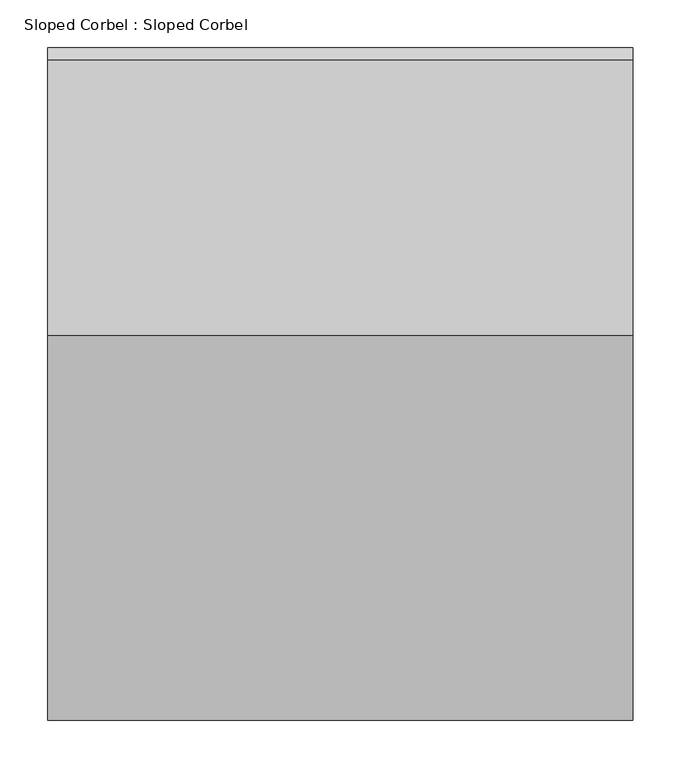
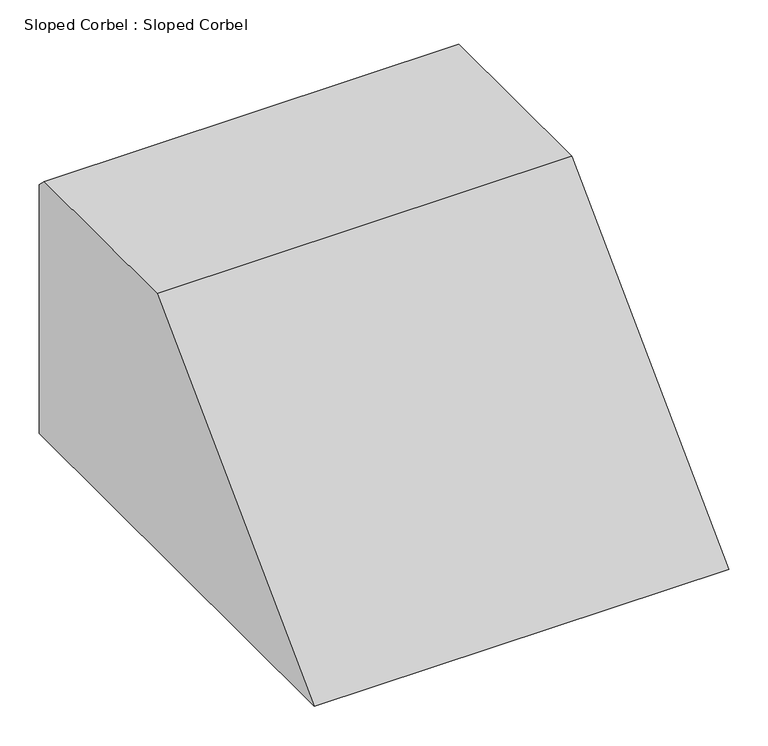
"""IFC4 building model written with IfcOpenShell, lengths in millimetres: fastener geometry, Sloped Corbel : Sloped Corbel."""

from ifc_helpers import new_model, si_unit, frame, origin, place, context, project, spatial, polyline, outline, extrude, source, transform, mapped, element, save


def sloped_corbel_sloped_corbel_c9660960(model_context):
    return source(origin(), model_context, "Body", "SweptSolid", [
        extrude(outline(polyline([(0.0, 387.3), (0.0, 0.0), (-700.0, 0.0), (-300.0, 400.0), (-12.7, 400.0), (0.0, 387.3)])), frame((-304.8, 0.0, 0.0), z_axis=(1.0, 0.0, 0.0), x_axis=(0.0, 1.0, 0.0)), (0.0, 0.0, 1.0), 609.6),
    ])


if __name__ == "__main__":
    model = new_model("IFC4")
    model_context = context("Model", 3, world=origin())
    ifc_project = project(units=[si_unit("LENGTHUNIT", "METRE", prefix="MILLI")], contexts=[model_context])
    site = spatial("IfcSite", under=ifc_project)
    building = spatial("IfcBuilding", under=site)
    placement = place(None, origin())
    sloped_corbel_sloped_corbel_shape = sloped_corbel_sloped_corbel_c9660960(model_context)
    element("IfcFastener", 1, ObjectType="Sloped Corbel : Sloped Corbel", at=placement, inside=building, context=model_context, shape_type="MappedRepresentation", body=[
        mapped(sloped_corbel_sloped_corbel_shape, transform((0.0, 0.0, 0.0), x_axis=(1.0, 0.0, 0.0), y_axis=(0.0, 1.0, 0.0), z_axis=(0.0, 0.0, 1.0))),
    ])
    save(model, "model.ifc")

# Revit data of these elements
# Project information
#   built-in parameter 1006321 = "Issue Date"
#   built-in parameter 1006320 = "Project Status"
#   built-in parameter 1006319 = "Owner"
#   built-in parameter 1006318 = "Enter address here"
#   built-in parameter 1006317 = "Project Name"
#   built-in parameter 1006316 = "Project Number"
# Type "Sloped Corbel : Sloped Corbel"
#   TransChamfer [instance default] = 0' - 0 1/2"
#   Corbel Width [instance default] = 1' - 0"
#   Corbel Height [instance default] = 2' - 3.55906"
#   Corbel Front [instance default] = 0' - 11.81102"
#   Corbel Depth [instance default] = 1' - 3.74803"
#   Chamfer = 0' - 0 1/2"
#   Material = Concrete - Precast Concrete - Normal Weight - 5 ksi
#   Default Elevation = 0
#   Assembly Code = ""
# Element 1 (IfcFastener, "Sloped Corbel : Sloped Corbel")
#   Corbel Width = 2' - 0"
#   Materials on its faces: "Concrete - Precast Concrete - Normal Weight - 5 ksi"
# Materials
#   "Concrete - Precast Concrete - Normal Weight - 5 ksi": class "Concrete", colour RGB 198 187 187, transparency 1
